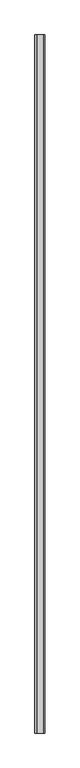
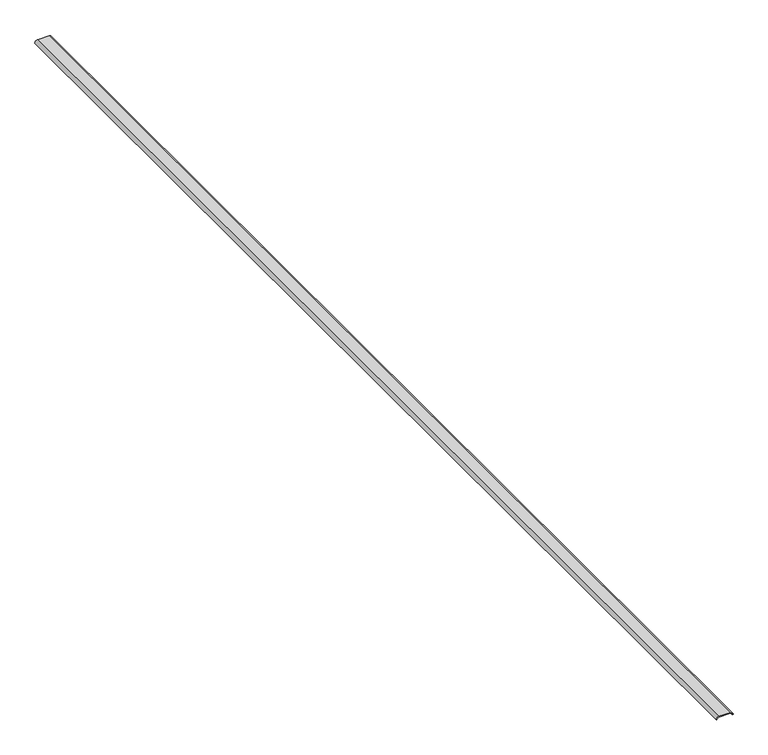
"""IFC4 building model written with IfcOpenShell, lengths in millimetres: proxy geometry, BEND PANEL004 6191 : BEND PANEL004 6191."""

from ifc_helpers import new_model, si_unit, point, frame, frame_2d, origin, place, context, project, spatial, polyline, circle_curve, trimmed, segment, composite_curve, outline, extrude, source, transform, mapped, element, save


def generic_models_15d214a6(model_context):
    return source(origin(), model_context, "Body", "SweptSolid", [
        extrude(outline(composite_curve([segment(polyline([(42576.61192, 5858.4004637), (42576.61192, 5859.5910887)]), True, "CONTINUOUS"), segment(trimmed(circle_curve(frame_2d((42576.6119199, 5862.9993652)), 3.4082764), [point((42576.61192, 5859.5910887))], [point((42580.0201795, 5863.0100787))], True, "CARTESIAN"), True, "CONTINUOUS"), segment(polyline([(42580.0201795, 5863.0100787), (42580.0201963, 5882.3645691)]), True, "CONTINUOUS"), segment(trimmed(circle_curve(frame_2d((42576.6119199, 5882.3645721)), 3.4082764), [point((42580.0201963, 5882.3645691))], [point((42576.61192, 5885.7728485))], True, "CARTESIAN"), True, "CONTINUOUS"), segment(polyline([(42576.61192, 5885.7728485), (42576.61192, 5886.9634735)]), True, "CONTINUOUS"), segment(trimmed(circle_curve(frame_2d((42576.6119199, 5882.3645721)), 4.5989014), [point((42576.61192, 5886.9634735))], [point((42581.2108213, 5882.364568))], False, "CARTESIAN"), True, "CONTINUOUS"), segment(polyline([(42581.2108213, 5882.364568), (42581.2108045, 5863.0118181)]), True, "CONTINUOUS"), segment(trimmed(circle_curve(frame_2d((42576.6119199, 5862.9993652)), 4.5989014), [point((42581.2108045, 5863.0118181))], [point((42576.61192, 5858.4004637))], False, "CARTESIAN"), True, "CONTINUOUS")], self_intersect=False)), frame((0.0, -1052.8906574, 0.0), z_axis=(0.0, 1.0, 0.0), x_axis=(0.0, 0.0, 1.0)), (0.0, 0.0, 1.0), 1999.85),
    ])


if __name__ == "__main__":
    model = new_model("IFC4")
    model_context = context("Model", 3, world=origin())
    ifc_project = project(units=[si_unit("LENGTHUNIT", "METRE", prefix="MILLI")], contexts=[model_context])
    site = spatial("IfcSite", under=ifc_project)
    building = spatial("IfcBuilding", under=site)
    placement = place(None, origin())
    generic_models_shape = generic_models_15d214a6(model_context)
    element("IfcBuildingElementProxy", 1, Name="BEND PANEL004 6191 : BEND PANEL004 6191", ObjectType="BEND PANEL004 6191 : BEND PANEL004 6191", at=placement, inside=building, context=model_context, shape_type="MappedRepresentation", body=[
        mapped(generic_models_shape, transform((0.0, 0.0, 0.0), x_axis=(1.0, 0.0, 0.0), y_axis=(0.0, 1.0, 0.0), z_axis=(0.0, 0.0, 1.0))),
    ])
    save(model, "model.ifc")

# Revit data of these elements
# Type "BEND PANEL004 6191 : BEND PANEL004 6191"
#   NameOverride = "BEND PANEL004"
# Element 1 (IfcBuildingElementProxy, "BEND PANEL004 6191 : BEND PANEL004 6191")
#   Materials on its faces: "METAL PROFILE"
# Materials
#   "METAL PROFILE": class "Unassigned", colour RGB 128 128 128, transparency 0
